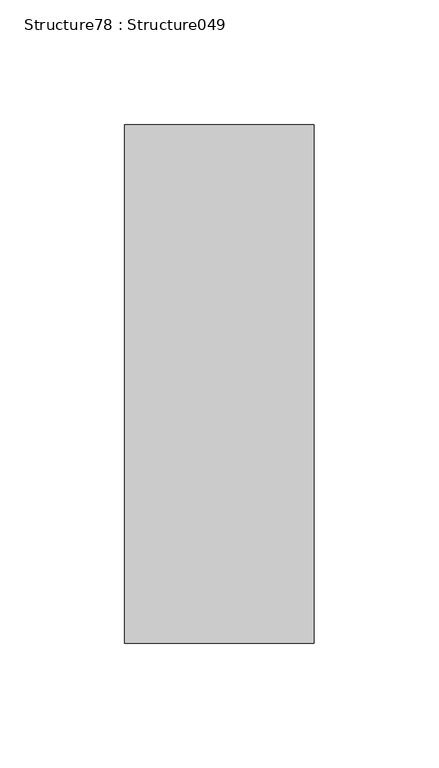
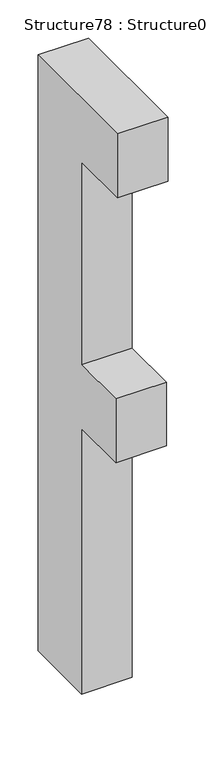
"""IFC4 building model written with IfcOpenShell, lengths in millimetres: proxy geometry, Structure78 : Structure049."""

from ifc_helpers import new_model, si_unit, frame, origin, place, context, project, spatial, polyline, outline, extrude, source, transform, mapped, element, save


def structure78_structure049_54f57d29(model_context):
    return source(origin(), model_context, "Body", "SweptSolid", [
        extrude(outline(polyline([(283060.9454638, 4480.4419946), (283060.9454638, 3528.5825142), (282946.7093274, 3528.5825142), (282946.7093274, 3952.8367913), (282856.9560968, 3952.8367913), (282856.9560968, 4054.8292705), (282946.7093274, 4054.8292705), (282946.7093274, 4378.4602217), (282852.888943, 4378.4602217), (282852.888943, 4480.4419946), (283060.9454638, 4480.4419946)])), frame((-59031.6926606, 0.0, 0.0), z_axis=(1.0, 0.0, 0.0), x_axis=(0.0, 1.0, 0.0)), (0.0, 0.0, 1.0), 76.2),
    ])


if __name__ == "__main__":
    model = new_model("IFC4")
    model_context = context("Model", 3, world=origin())
    ifc_project = project(units=[si_unit("LENGTHUNIT", "METRE", prefix="MILLI")], contexts=[model_context])
    site = spatial("IfcSite", under=ifc_project)
    building = spatial("IfcBuilding", under=site)
    placement = place(None, origin())
    structure78_structure049_shape = structure78_structure049_54f57d29(model_context)
    element("IfcBuildingElementProxy", 1, Name="Structure78 : Structure049", ObjectType="Structure78 : Structure049", at=placement, inside=building, context=model_context, shape_type="MappedRepresentation", body=[
        mapped(structure78_structure049_shape, transform((0.0, 0.0, 0.0), x_axis=(1.0, 0.0, 0.0), y_axis=(0.0, 1.0, 0.0), z_axis=(0.0, 0.0, 1.0))),
    ])
    save(model, "model.ifc")

# Revit data of these elements
# Type "Structure78 : Structure049"
#   NameOverride = "Structure049"
# Element 1 (IfcBuildingElementProxy, "Structure78 : Structure049")
#   Materials on its faces: "BRUSHED ALUM. LETTERING"
# Materials
#   "BRUSHED ALUM. LETTERING": class "Unassigned", colour RGB 169 181 186, transparency 0, Cost = 0
